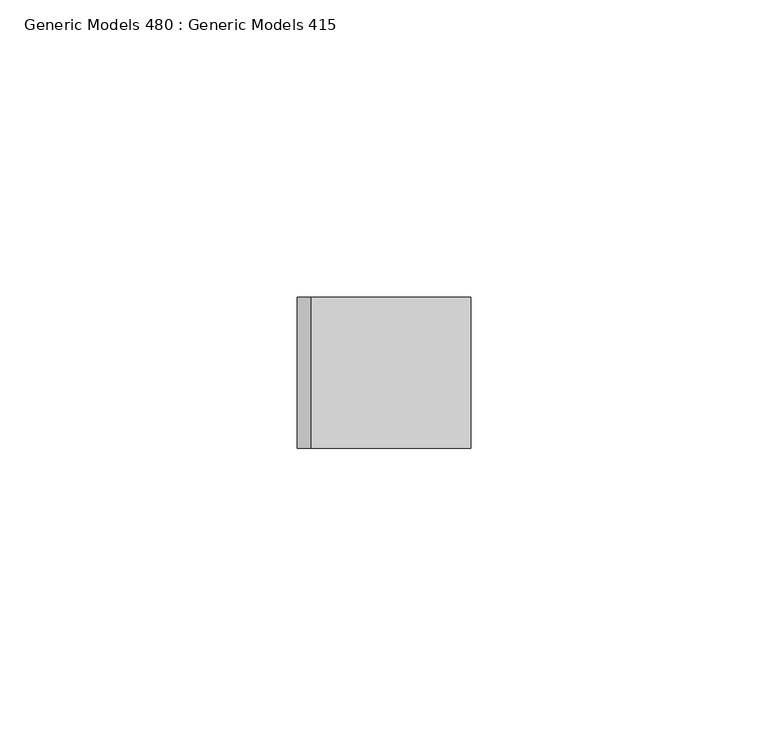
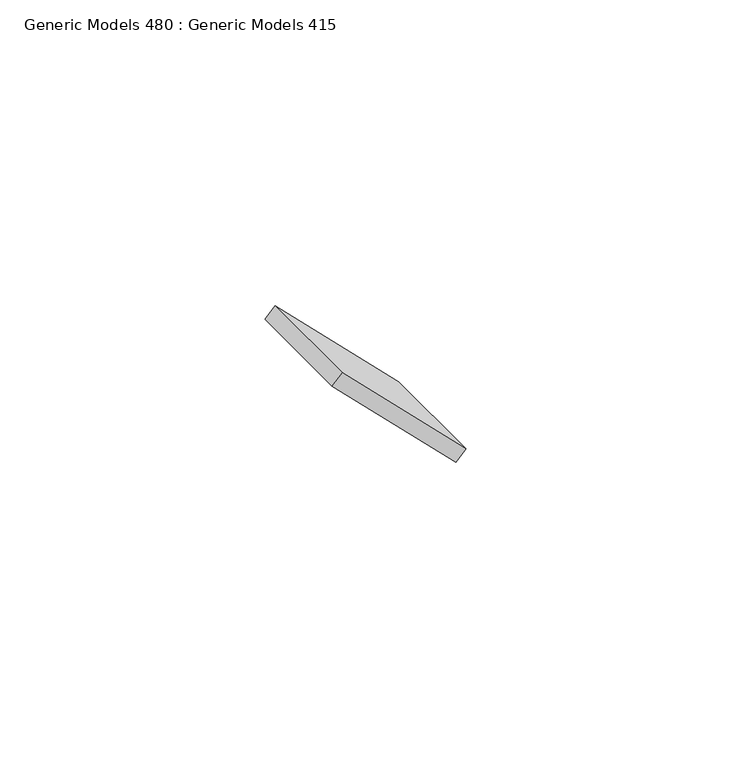
"""IFC4 building model written with IfcOpenShell, lengths in millimetres: proxy geometry, Generic Models 480 : Generic Models 415."""

from ifc_helpers import new_model, si_unit, frame, origin, place, context, project, spatial, polyline, outline, extrude, source, transform, mapped, element, save


def generic_models_480_generic_models_415_16ca8967(model_context):
    return source(origin(), model_context, "Body", "SweptSolid", [
        extrude(outline(polyline([(0.0, -38.1), (0.0, 0.0), (25.4, 0.0), (25.4, -38.1), (0.0, -38.1)])), frame((-6869.8996186, -4475.9863946, 127845.0002957), z_axis=(0.7071067811864907, 0.0, 0.7071067811866044), x_axis=(0.0, -1.0, 0.0)), (0.0, 0.0, 1.0), 3.175),
    ])


if __name__ == "__main__":
    model = new_model("IFC4")
    model_context = context("Model", 3, world=origin())
    ifc_project = project(units=[si_unit("LENGTHUNIT", "METRE", prefix="MILLI")], contexts=[model_context])
    site = spatial("IfcSite", under=ifc_project)
    building = spatial("IfcBuilding", under=site)
    placement = place(None, origin())
    generic_models_480_generic_models_415_shape = generic_models_480_generic_models_415_16ca8967(model_context)
    element("IfcBuildingElementProxy", 1, Name="Generic Models 480 : Generic Models 415", ObjectType="Generic Models 480 : Generic Models 415", at=placement, inside=building, context=model_context, shape_type="MappedRepresentation", body=[
        mapped(generic_models_480_generic_models_415_shape, transform((0.0, 0.0, 0.0), x_axis=(1.0, 0.0, 0.0), y_axis=(0.0, 1.0, 0.0), z_axis=(0.0, 0.0, 1.0))),
    ])
    save(model, "model.ifc")

# Revit data of these elements
# Element 1 (IfcBuildingElementProxy, "Generic Models 480 : Generic Models 415")
#   Materials on its faces: "_WELDED STEEL TABS FOR LOUVER ATTACHMENT"
# Materials
#   "_WELDED STEEL TABS FOR LOUVER ATTACHMENT": class "Metal", colour RGB 199 199 199, transparency 0, Description = "Structural steel 50ksi", Cost = 0
